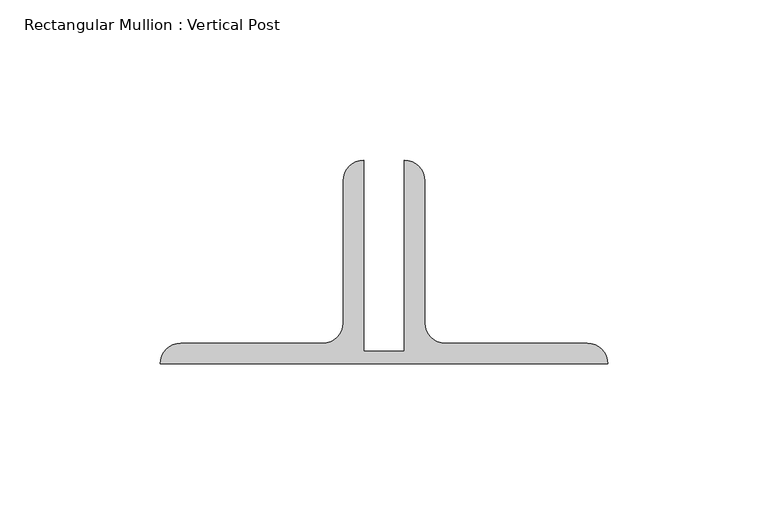
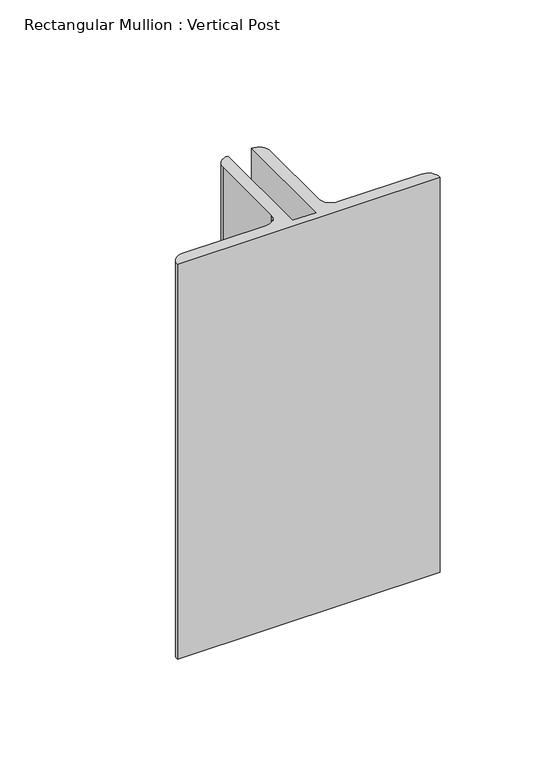
"""IFC4 building model written with IfcOpenShell, lengths in millimetres: member geometry, Rectangular Mullion : Vertical Post."""

from ifc_helpers import new_model, si_unit, point, frame, frame_2d, origin, place, context, project, spatial, polyline, circle_curve, trimmed, segment, composite_curve, outline, extrude, source, transform, mapped, element, save


def rectangular_mullion_vertical_post_0441d5d9(model_context):
    return source(origin(), model_context, "Body", "SweptSolid", [
        extrude(outline(composite_curve([segment(polyline([(-63.5, 22.9145205), (-63.5, 82.55)]), True, "CONTINUOUS"), segment(trimmed(circle_curve(frame_2d((-63.5, 76.2)), 6.35), [point((-63.5, 82.55))], [point((-57.15, 76.2))], False, "CARTESIAN"), True, "CONTINUOUS"), segment(polyline([(-57.15, 76.2), (-57.15, 31.75)]), True, "CONTINUOUS"), segment(trimmed(circle_curve(frame_2d((-50.8, 31.75)), 6.35), [point((-57.15, 31.75))], [point((-50.8, 25.4))], True, "CARTESIAN"), True, "CONTINUOUS"), segment(polyline([(-50.8, 25.4), (-6.35, 25.4)]), True, "CONTINUOUS"), segment(trimmed(circle_curve(frame_2d((-6.35, 19.05)), 6.35), [point((-6.35, 25.4))], [point((0.0, 19.05))], False, "CARTESIAN"), True, "CONTINUOUS"), segment(polyline([(0.0, 19.05), (-139.7, 19.05)]), True, "CONTINUOUS"), segment(trimmed(circle_curve(frame_2d((-133.35, 19.05)), 6.35), [point((-139.7, 19.05))], [point((-133.35, 25.4))], False, "CARTESIAN"), True, "CONTINUOUS"), segment(polyline([(-133.35, 25.4), (-88.9, 25.4)]), True, "CONTINUOUS"), segment(trimmed(circle_curve(frame_2d((-88.9, 31.75)), 6.35), [point((-88.9, 25.4))], [point((-82.55, 31.75))], True, "CARTESIAN"), True, "CONTINUOUS"), segment(polyline([(-82.55, 31.75), (-82.55, 76.2)]), True, "CONTINUOUS"), segment(trimmed(circle_curve(frame_2d((-76.2, 76.2)), 6.35), [point((-82.55, 76.2))], [point((-76.2, 82.55))], False, "CARTESIAN"), True, "CONTINUOUS"), segment(polyline([(-76.2, 82.55), (-76.2, 22.9145205), (-63.5, 22.9145205)]), True, "CONTINUOUS")], self_intersect=False)), frame((0.0, 0.0, -222.0889998), z_axis=(0.0, 0.0, 1.0), x_axis=(1.0, 0.0, 0.0)), (0.0, 0.0, 1.0), 222.0889998),
    ])


if __name__ == "__main__":
    model = new_model("IFC4")
    model_context = context("Model", 3, world=origin())
    ifc_project = project(units=[si_unit("LENGTHUNIT", "METRE", prefix="MILLI")], contexts=[model_context])
    site = spatial("IfcSite", under=ifc_project)
    building = spatial("IfcBuilding", under=site)
    placement = place(None, origin())
    rectangular_mullion_vertical_post_shape = rectangular_mullion_vertical_post_0441d5d9(model_context)
    element("IfcMember", 1, ObjectType="Rectangular Mullion : Vertical Post", at=placement, inside=building, context=model_context, shape_type="MappedRepresentation", body=[
        mapped(rectangular_mullion_vertical_post_shape, transform((0.0, 0.0, 0.0), x_axis=(1.0, 0.0, 0.0), y_axis=(0.0, 1.0, 0.0), z_axis=(0.0, 0.0, 1.0))),
    ])
    save(model, "model.ifc")

# Revit data of these elements
# Type "Rectangular Mullion : Vertical Post"
#   built-in parameter 1007351 = -0.0625 (stored number, unit not read)
#   built-in parameter 1007322 = 0.0126789 (stored number, unit not read)
#   built-in parameter 1007321 = 0.229167 (stored number, unit not read)
#   built-in parameter 1007320 = 0.229167 (stored number, unit not read)
# Element 1 (IfcMember, "Rectangular Mullion : Vertical Post")
#   Materials on its faces: "GATE POST: (2) BACK/BACK GALVANIZED ANGLES"
# Materials
#   "GATE POST: (2) BACK/BACK GALVANIZED ANGLES": class "Unassigned", colour RGB 211 211 211, transparency 0, Cost = 0
